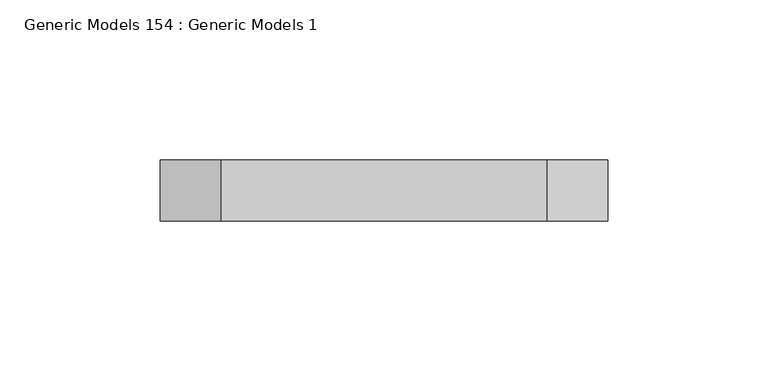
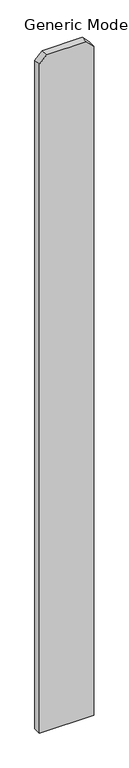
"""IFC4 building model written with IfcOpenShell, lengths in millimetres: proxy geometry, Generic Models 154 : Generic Models 1."""

from ifc_helpers import new_model, si_unit, frame, origin, place, context, project, spatial, polyline, outline, extrude, source, transform, mapped, element, save


def generic_models_154_generic_models_1_06d36a19(model_context):
    return source(origin(), model_context, "Body", "SweptSolid", [
        extrude(outline(polyline([(76.2, 53922.6125), (1885.95, 53922.6125), (1905.0, 53903.5625), (1905.0, 53801.9625), (1885.95, 53782.9125), (76.2, 53782.9125), (76.2, 53922.6125)])), frame((0.0, 547.6875, 0.0), z_axis=(0.0, 1.0, 0.0), x_axis=(0.0, 0.0, 1.0)), (0.0, 0.0, 1.0), 19.05),
    ])


if __name__ == "__main__":
    model = new_model("IFC4")
    model_context = context("Model", 3, world=origin())
    ifc_project = project(units=[si_unit("LENGTHUNIT", "METRE", prefix="MILLI")], contexts=[model_context])
    site = spatial("IfcSite", under=ifc_project)
    building = spatial("IfcBuilding", under=site)
    placement = place(None, origin())
    generic_models_154_generic_models_1_shape = generic_models_154_generic_models_1_06d36a19(model_context)
    element("IfcBuildingElementProxy", 1, Name="Generic Models 154 : Generic Models 1", ObjectType="Generic Models 154 : Generic Models 1", at=placement, inside=building, context=model_context, shape_type="MappedRepresentation", body=[
        mapped(generic_models_154_generic_models_1_shape, transform((0.0, 0.0, 0.0), x_axis=(1.0, 0.0, 0.0), y_axis=(0.0, 1.0, 0.0), z_axis=(0.0, 0.0, 1.0))),
    ])
    save(model, "model.ifc")

# Revit data of these elements
# Element 1 (IfcBuildingElementProxy, "Generic Models 154 : Generic Models 1")
#   Materials on its faces: "VERTICAL 1X6 CEDAR PLANKS W/ CLEAR WOOD SEALER"
# Materials
#   "VERTICAL 1X6 CEDAR PLANKS W/ CLEAR WOOD SEALER": class "Wood", colour RGB 234 198 147, transparency 0, Description = "Pinus Echinata", Cost = 0
